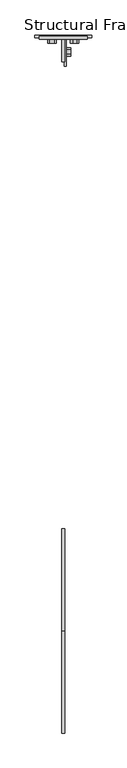
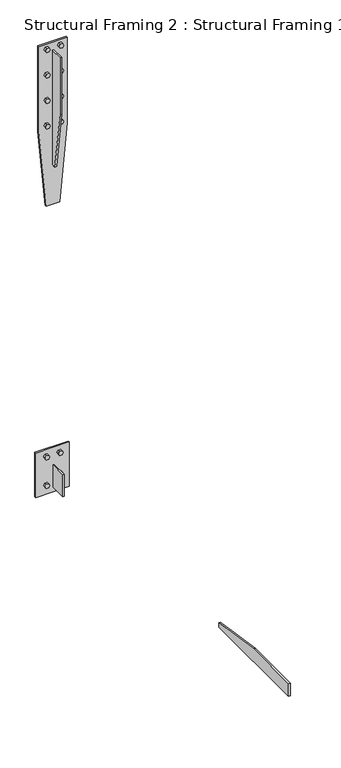
"""IFC4 building model written with IfcOpenShell, lengths in millimetres: beam geometry, Structural Framing 2 : Structural Framing 1."""

from ifc_helpers import new_model, si_unit, frame, origin, place, context, project, spatial, polyline, outline, extrude, source, transform, mapped, element, save


def structural_framing_2_structural_framing_1_fc76d0cb(model_context):
    return source(origin(), model_context, "Body", "SweptSolid", [
        extrude(outline(polyline([(-74.0021465, 3361.7022161), (-93.0521465, 3361.7022161), (-102.5771465, 3378.2), (-93.0521465, 3394.6977839), (-74.0021465, 3394.6977839), (-64.4771465, 3378.2), (-74.0021465, 3361.7022161)])), frame((-9182.1913771, 0.0, 0.0), z_axis=(1.0, 0.0, 0.0), x_axis=(0.0, 1.0, 0.0)), (0.0, 0.0, 1.0), 19.05),
        extrude(outline(polyline([(-74.0021465, 3295.1297839), (-64.4771465, 3278.632), (-74.0021465, 3262.1342161), (-93.0521465, 3262.1342161), (-102.5771465, 3278.632), (-93.0521465, 3295.1297839), (-74.0021465, 3295.1297839)])), frame((-9182.1913771, 0.0, 0.0), z_axis=(1.0, 0.0, 0.0), x_axis=(0.0, 1.0, 0.0)), (0.0, 0.0, 1.0), 19.05),
        extrude(outline(polyline([(-9182.1913771, -147.0271465), (-9191.7163771, -147.0271465), (-9191.7163771, -20.0271465), (-9182.1913771, -20.0271465), (-9182.1913771, -147.0271465)])), frame((0.0, 0.0, 3239.516), z_axis=(0.0, 0.0, 1.0), x_axis=(1.0, 0.0, 0.0)), (0.0, 0.0, 1.0), 177.8),
        extrude(outline(polyline([(3295.1297839, -9256.0418771), (3278.632, -9265.5668771), (3262.1342161, -9256.0418771), (3262.1342161, -9236.9918771), (3278.632, -9227.4668771), (3295.1297839, -9236.9918771), (3295.1297839, -9256.0418771)])), frame((0.0, -39.0771465, 0.0), z_axis=(0.0, 1.0, 0.0), x_axis=(0.0, 0.0, 1.0)), (0.0, 0.0, 1.0), 19.05),
        extrude(outline(polyline([(3523.7297839, -9256.0418771), (3507.232, -9265.5668771), (3490.7342161, -9256.0418771), (3490.7342161, -9236.9918771), (3507.232, -9227.4668771), (3523.7297839, -9236.9918771), (3523.7297839, -9256.0418771)])), frame((0.0, -39.0771465, 0.0), z_axis=(0.0, 1.0, 0.0), x_axis=(0.0, 0.0, 1.0)), (0.0, 0.0, 1.0), 19.05),
        extrude(outline(polyline([(3295.1297839, -9135.3918771), (3295.1297839, -9154.4418771), (3278.632, -9163.9668771), (3262.1342161, -9154.4418771), (3262.1342161, -9135.3918771), (3278.632, -9125.8668771), (3295.1297839, -9135.3918771)])), frame((0.0, -39.0771465, 0.0), z_axis=(0.0, 1.0, 0.0), x_axis=(0.0, 0.0, 1.0)), (0.0, 0.0, 1.0), 19.05),
        extrude(outline(polyline([(3523.7297839, -9135.3918771), (3523.7297839, -9154.4418771), (3507.232, -9163.9668771), (3490.7342161, -9154.4418771), (3490.7342161, -9135.3918771), (3507.232, -9125.8668771), (3523.7297839, -9135.3918771)])), frame((0.0, -39.0771465, 0.0), z_axis=(0.0, 1.0, 0.0), x_axis=(0.0, 0.0, 1.0)), (0.0, 0.0, 1.0), 19.05),
        extrude(outline(polyline([(-9322.7168771, -7.3271465), (-9068.7168771, -7.3271465), (-9068.7168771, -20.0271465), (-9322.7168771, -20.0271465), (-9322.7168771, -7.3271465)])), frame((0.0, 0.0, 3202.432), z_axis=(0.0, 0.0, 1.0), x_axis=(1.0, 0.0, 0.0)), (0.0, 0.0, 1.0), 355.6),
        extrude(outline(polyline([(6175.9977839, -9236.9918771), (6175.9977839, -9256.0418771), (6159.5, -9265.5668771), (6143.0022161, -9256.0418771), (6143.0022161, -9236.9918771), (6159.5, -9227.4668771), (6175.9977839, -9236.9918771)])), frame((0.0, -45.4271465, 0.0), z_axis=(0.0, 1.0, 0.0), x_axis=(0.0, 0.0, 1.0)), (0.0, 0.0, 1.0), 19.05),
        extrude(outline(polyline([(6175.9977839, -9135.3918771), (6175.9977839, -9154.4418771), (6159.5, -9163.9668771), (6143.0022161, -9154.4418771), (6143.0022161, -9135.3918771), (6159.5, -9125.8668771), (6175.9977839, -9135.3918771)])), frame((0.0, -45.4271465, 0.0), z_axis=(0.0, 1.0, 0.0), x_axis=(0.0, 0.0, 1.0)), (0.0, 0.0, 1.0), 19.05),
        extrude(outline(polyline([(6379.1977839, -9236.9918771), (6379.1977839, -9256.0418771), (6362.7, -9265.5668771), (6346.2022161, -9256.0418771), (6346.2022161, -9236.9918771), (6362.7, -9227.4668771), (6379.1977839, -9236.9918771)])), frame((0.0, -45.4271465, 0.0), z_axis=(0.0, 1.0, 0.0), x_axis=(0.0, 0.0, 1.0)), (0.0, 0.0, 1.0), 19.05),
        extrude(outline(polyline([(6379.1977839, -9135.3918771), (6379.1977839, -9154.4418771), (6362.7, -9163.9668771), (6346.2022161, -9154.4418771), (6346.2022161, -9135.3918771), (6362.7, -9125.8668771), (6379.1977839, -9135.3918771)])), frame((0.0, -45.4271465, 0.0), z_axis=(0.0, 1.0, 0.0), x_axis=(0.0, 0.0, 1.0)), (0.0, 0.0, 1.0), 19.05),
        extrude(outline(polyline([(6582.3977839, -9236.9918771), (6582.3977839, -9256.0418771), (6565.9, -9265.5668771), (6549.4022161, -9256.0418771), (6549.4022161, -9236.9918771), (6565.9, -9227.4668771), (6582.3977839, -9236.9918771)])), frame((0.0, -45.4271465, 0.0), z_axis=(0.0, 1.0, 0.0), x_axis=(0.0, 0.0, 1.0)), (0.0, 0.0, 1.0), 19.05),
        extrude(outline(polyline([(6582.3977839, -9135.3918771), (6582.3977839, -9154.4418771), (6565.9, -9163.9668771), (6549.4022161, -9154.4418771), (6549.4022161, -9135.3918771), (6565.9, -9125.8668771), (6582.3977839, -9135.3918771)])), frame((0.0, -45.4271465, 0.0), z_axis=(0.0, 1.0, 0.0), x_axis=(0.0, 0.0, 1.0)), (0.0, 0.0, 1.0), 19.05),
        extrude(outline(polyline([(6785.5977839, -9236.9918771), (6785.5977839, -9256.0418771), (6769.1, -9265.5668771), (6752.6022161, -9256.0418771), (6752.6022161, -9236.9918771), (6769.1, -9227.4668771), (6785.5977839, -9236.9918771)])), frame((0.0, -45.4271465, 0.0), z_axis=(0.0, 1.0, 0.0), x_axis=(0.0, 0.0, 1.0)), (0.0, 0.0, 1.0), 19.05),
        extrude(outline(polyline([(6785.5977839, -9135.3918771), (6785.5977839, -9154.4418771), (6769.1, -9163.9668771), (6752.6022161, -9154.4418771), (6752.6022161, -9135.3918771), (6769.1, -9125.8668771), (6785.5977839, -9135.3918771)])), frame((0.0, -45.4271465, 0.0), z_axis=(0.0, 1.0, 0.0), x_axis=(0.0, 0.0, 1.0)), (0.0, 0.0, 1.0), 19.05),
        extrude(outline(polyline([(-3128.0411296, 3556.0), (-2670.8411296, 3556.0), (-2213.6411296, 3488.6697466), (-2213.6411296, 3454.4), (-3128.0411296, 3454.4), (-3128.0411296, 3556.0)])), frame((-9202.0668771, 0.0, 0.0), z_axis=(1.0, 0.0, 0.0), x_axis=(0.0, 1.0, 0.0)), (0.0, 0.0, 1.0), 12.7),
        extrude(outline(polyline([(-127.9771465, 6743.7), (-26.3771465, 6743.7), (-26.3771465, 5829.3), (-60.6468931, 5829.3), (-127.9771465, 6286.5), (-127.9771465, 6743.7)])), frame((-9202.0668771, 0.0, 0.0), z_axis=(1.0, 0.0, 0.0), x_axis=(0.0, 1.0, 0.0)), (0.0, 0.0, 1.0), 12.7),
        extrude(outline(polyline([(6121.4, -9303.6668771), (5511.8, -9246.5168771), (5511.8, -9144.9168771), (6121.4, -9087.7668771), (6807.2, -9087.7668771), (6807.2, -9303.6668771), (6121.4, -9303.6668771)])), frame((0.0, -26.3771465, 0.0), z_axis=(0.0, 1.0, 0.0), x_axis=(0.0, 0.0, 1.0)), (0.0, 0.0, 1.0), 12.7),
    ])


if __name__ == "__main__":
    model = new_model("IFC4")
    model_context = context("Model", 3, world=origin())
    ifc_project = project(units=[si_unit("LENGTHUNIT", "METRE", prefix="MILLI")], contexts=[model_context])
    site = spatial("IfcSite", under=ifc_project)
    building = spatial("IfcBuilding", under=site)
    placement = place(None, origin())
    structural_framing_2_structural_framing_1_shape = structural_framing_2_structural_framing_1_fc76d0cb(model_context)
    element("IfcBeam", 1, ObjectType="Structural Framing 2 : Structural Framing 1", at=placement, inside=building, context=model_context, shape_type="MappedRepresentation", body=[
        mapped(structural_framing_2_structural_framing_1_shape, transform((0.0, 0.0, 0.0), x_axis=(1.0, 0.0, 0.0), y_axis=(0.0, 1.0, 0.0), z_axis=(0.0, 0.0, 1.0))),
    ])
    save(model, "model.ifc")

# Revit data of these elements
# Element 1 (IfcBeam, "Structural Framing 2 : Structural Framing 1")
#   Materials on its faces: "Galvanized Steel"
# Materials
#   "Galvanized Steel": class "Generic", colour RGB 232 232 232, transparency 0, Description = "Acoustic Ceiling Tile 24 x 24", Cost = 0
